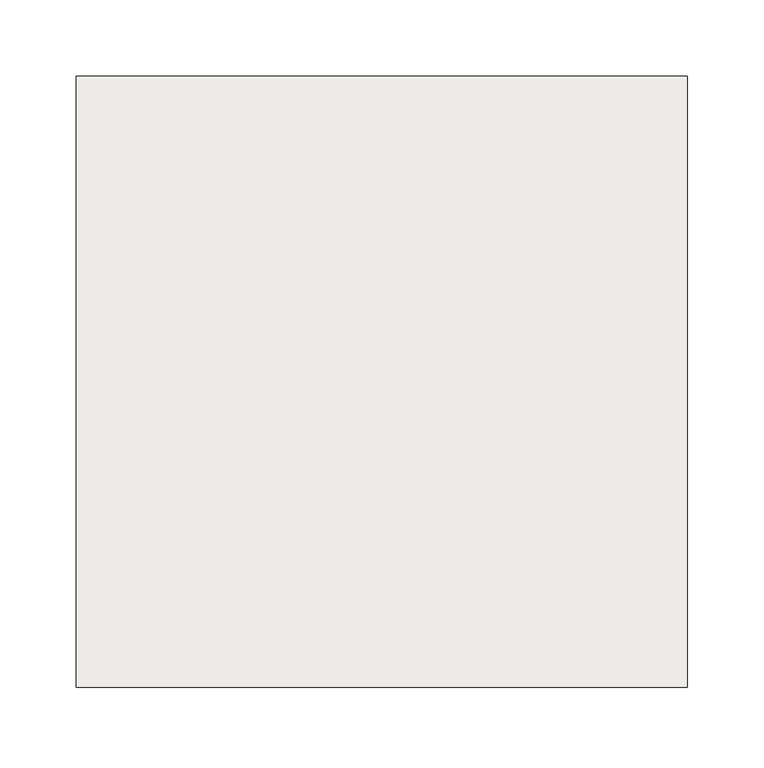
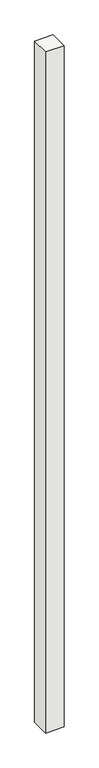
"""IFC4 building model written with IfcOpenShell, lengths in millimetres: footing geometry, NLRS_17_SFO_TLB_funderingspaal geheid beton prefab-AV-MMBPC_gen_rsf : heipaal beton prefab_gen__bxh 400x400."""

from ifc_helpers import new_model, si_unit, frame, origin, place, context, project, spatial, polyline, outline, extrude, source, transform, mapped, element, save


def footing_4eaa82be(model_context):
    return source(origin(), model_context, "Body", "SweptSolid", [
        extrude(outline(polyline([(200.0, -200.0), (-200.0, -200.0), (-200.0, 200.0), (200.0, 200.0), (200.0, -200.0)])), frame((0.0, 0.0, -20000.0), z_axis=(0.0, 0.0, 1.0), x_axis=(1.0, 0.0, 0.0)), (0.0, 0.0, 1.0), 15520.0),
    ])


if __name__ == "__main__":
    model = new_model("IFC4")
    model_context = context("Model", 3, world=origin())
    ifc_project = project(units=[si_unit("LENGTHUNIT", "METRE", prefix="MILLI")], contexts=[model_context])
    site = spatial("IfcSite", under=ifc_project)
    building = spatial("IfcBuilding", under=site)
    placement = place(None, origin())
    footing_shape = footing_4eaa82be(model_context)
    element("IfcFooting", 1, ObjectType="NLRS_17_SFO_TLB_funderingspaal geheid beton prefab-AV-MMBPC_gen_rsf : heipaal beton prefab_gen__bxh 400x400", at=placement, inside=building, context=model_context, shape_type="MappedRepresentation", body=[
        mapped(footing_shape, transform((0.0, 0.0, 0.0), x_axis=(1.0, 0.0, 0.0), y_axis=(0.0, 1.0, 0.0), z_axis=(0.0, 0.0, 1.0))),
    ])
    save(model, "model.ifc")

# Revit data of these elements
# Type "NLRS_17_SFO_TLB_funderingspaal geheid beton prefab-AV-MMBPC_gen_rsf : heipaal beton prefab_gen__bxh 400x400"
#   IfcExportAs = "IfcPile"
#   Type Comments = "prefab heipaal 400x400"
#   Model = " "
#   Manufacturer = " "
#   Description = "prefab heipaal 400x400"
#   Assembly Code = "17.21"
#   Width = 400 mm
#   Slanted Angle [instance default] = 0.00°
#   NLRS_S_draagvermogen_trek [instance default] = 0.00 kN
#   NLRS_S_draagvermogen_druk [instance default] = 0.00 kN
#   NLRS_C_lengte [instance default] = 1660 mm
#   NLRS_C_hoogte = 400 mm
#   NLRS_C_breedte = 400 mm
#   Height [instance default] = 1660 mm
#   Length [instance default] = 1660 mm
#   Angle [instance default] = 0.00°
#   Slanted [instance default] = 0
#   Structural Material = NLRS_f2_beton prefab_gen_rsf
#   Keynote = ""
# Element 1 (IfcFooting, "NLRS_17_SFO_TLB_funderingspaal geheid beton prefab-AV-MMBPC_gen_rsf : heipaal beton prefab_gen__bxh 400x400")
#   NLRS_C_lengte = 15520 mm
#   Height = 15520 mm
#   Length = 15520 mm
#   Materials on its faces: "NLRS_f2_beton prefab_gen_rsf"
# Materials
#   "NLRS_f2_beton prefab_gen_rsf": class "F - Niet gebakken kunststeen", colour RGB 129 133 118, transparency 0, Keynote = "f2", Manufacturer = "Revit Standards Foundation", URL = "www.revitstandards.org", Description = "beton prefab", Cost = 0
